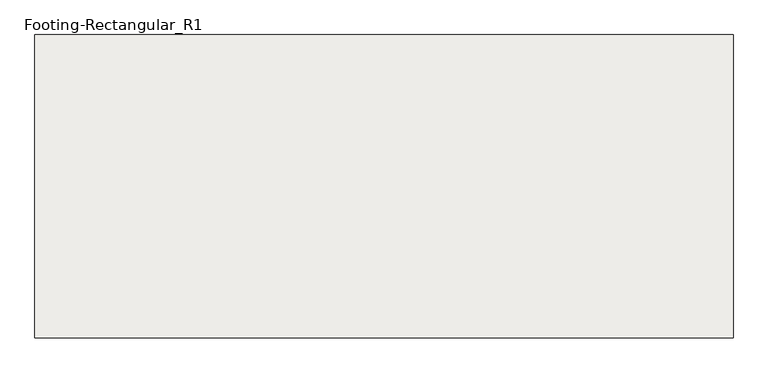
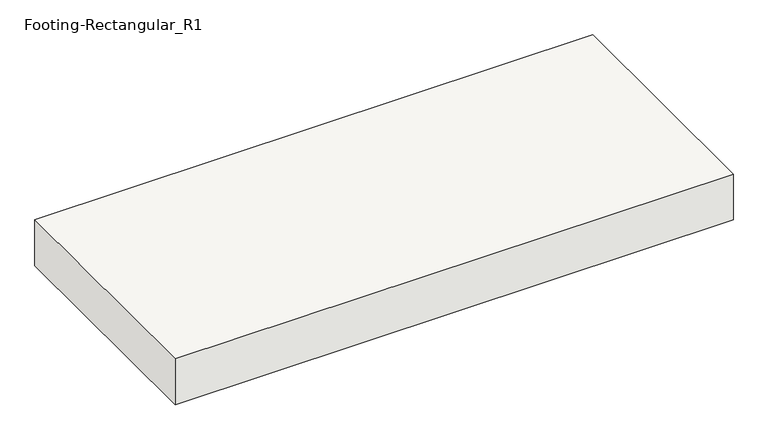
"""IFC4 building model written with IfcOpenShell, lengths in millimetres: slab geometry, Footing-Rectangular_R1 : H_SF_AR_S18_W5750xL2500xT500_Bitumen_F6."""

from ifc_helpers import new_model, si_unit, frame, origin, place, context, project, spatial, polyline, outline, extrude, source, transform, mapped, element, save


def footing_rectangular_r1_f7e30f5b(model_context):
    return source(origin(), model_context, "Body", "SweptSolid", [
        extrude(outline(polyline([(2875.0, 1250.0), (2875.0, -1250.0), (-2875.0, -1250.0), (-2875.0, 1250.0), (2875.0, 1250.0)])), frame((0.0, 0.0, -500.0), z_axis=(0.0, 0.0, 1.0), x_axis=(1.0, 0.0, 0.0)), (0.0, 0.0, 1.0), 500.0),
    ])


if __name__ == "__main__":
    model = new_model("IFC4")
    model_context = context("Model", 3, world=origin())
    ifc_project = project(units=[si_unit("LENGTHUNIT", "METRE", prefix="MILLI")], contexts=[model_context])
    site = spatial("IfcSite", under=ifc_project)
    building = spatial("IfcBuilding", under=site)
    placement = place(None, origin())
    footing_rectangular_r1_shape = footing_rectangular_r1_f7e30f5b(model_context)
    element("IfcSlab", 1, ObjectType="Footing-Rectangular_R1 : H_SF_AR_S18_W5750xL2500xT500_Bitumen_F6", at=placement, inside=building, context=model_context, shape_type="MappedRepresentation", body=[
        mapped(footing_rectangular_r1_shape, transform((0.0, 0.0, 0.0), x_axis=(1.0, 0.0, 0.0), y_axis=(0.0, 1.0, 0.0), z_axis=(0.0, 0.0, 1.0))),
    ])
    save(model, "model.ifc")

# Revit data of these elements
# Type "Footing-Rectangular_R1 : H_SF_AR_S18_W5750xL2500xT500_Bitumen_F6"
#   Type Mark = "F6"
#   Top bar = "D25@300"
#   Description = "UG Shallow Foundation"
#   Bottom bar = "D20@300"
#   Width = 5750 mm
#   Length = 2500 mm
#   Foundation Thickness = 500 mm
#   Structural Material [instance default] = none
#   Assembly Code = ""
